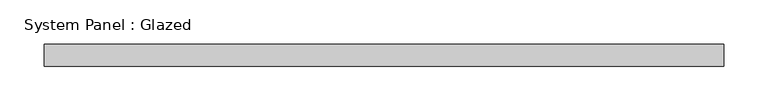
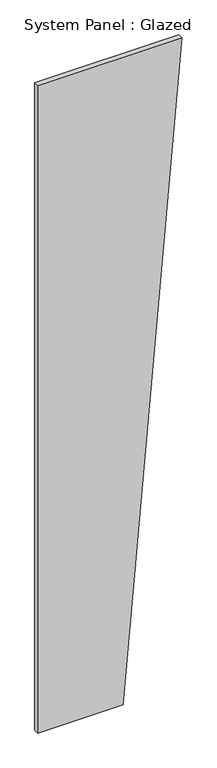
"""IFC4 building model written with IfcOpenShell, lengths in millimetres: plate geometry, System Panel : Glazed."""

import ifcopenshell
import ifcopenshell.guid

model = None  # the IFC model being written
_history = None  # IfcOwnerHistory: only IFC2X3 demands one
_inside = {}  # id of a spatial element -> (the spatial element, [elements in it])
_under = {}  # id of a project, library or spatial element -> (it, [spatial elements below it])
_declared = {}  # id of a project -> (the project, [libraries it declares])
_typed = {}  # id of a type object -> (the type object, [elements of that type])
_made_of = {}  # id of a material, layer set ... -> (it, [elements and type objects made of it])


def new_model(schema):
    """Start an empty IFC model of exactly this schema.

    Asked for "IFC4X3", IfcOpenShell would pick the latest addendum, in which some entities
    have other attributes; the version numbers below select the first issue.
    IFC2X3 requires an IfcOwnerHistory on every rooted entity: one is made here for all.
    """
    global model, _history
    if schema == "IFC4X3":
        model = ifcopenshell.file(schema_version=(4, 3, 0, 0))
    else:
        model = ifcopenshell.file(schema=schema)
    _inside.clear()
    _under.clear()
    _declared.clear()
    _typed.clear()
    _made_of.clear()
    _history = None
    if model.schema == "IFC2X3":
        org = make("IfcOrganization", Name="unknown")
        user = make(
            "IfcPersonAndOrganization",
            ThePerson=make("IfcPerson", FamilyName="unknown"),
            TheOrganization=org,
        )
        app = make(
            "IfcApplication",
            ApplicationDeveloper=org,
            Version="unknown",
            ApplicationFullName="unknown",
            ApplicationIdentifier="unknown",
        )
        _history = make(
            "IfcOwnerHistory",
            OwningUser=user,
            OwningApplication=app,
            ChangeAction="ADDED",
            CreationDate=0,
        )
    return model


def make(cls, **values):
    """One entity of the class cls with the attributes given. An attribute that is None is left unset."""
    return model.create_entity(
        cls, **{name: value for name, value in values.items() if value is not None}
    )


def rooted(cls, **values):
    """An entity with a GlobalId (a new one), such as an element, a storey or a relation."""
    return make(cls, GlobalId=ifcopenshell.guid.new(), OwnerHistory=_history, **values)


def si_unit(unit_type, name, prefix=None):
    """IfcSIUnit, for example si_unit("LENGTHUNIT", "METRE", prefix="MILLI")."""
    return make("IfcSIUnit", UnitType=unit_type, Prefix=prefix, Name=name)


def assignment(units):
    """IfcUnitAssignment: the units of a project."""
    return None if units is None else make("IfcUnitAssignment", Units=units)


def point(xyz):
    """IfcCartesianPoint."""
    return None if xyz is None else make("IfcCartesianPoint", Coordinates=xyz)


def direction(xyz):
    """IfcDirection."""
    return None if xyz is None else make("IfcDirection", DirectionRatios=xyz)


def frame(location, z_axis=None, x_axis=None):
    """IfcAxis2Placement3D, a coordinate frame: its origin and axes. An axis left out is left unset."""
    return make(
        "IfcAxis2Placement3D",
        Location=point(location),
        Axis=direction(z_axis),
        RefDirection=direction(x_axis),
    )


def origin():
    """The frame at (0, 0, 0) with its axes left unset."""
    return frame((0.0, 0.0, 0.0))


def place(relative_to, where):
    """IfcLocalPlacement: puts the frame where relative to a parent placement (None: the world)."""
    return make(
        "IfcLocalPlacement", PlacementRelTo=relative_to, RelativePlacement=where
    )


def context(
    kind, dimensions, precision=None, world=None, true_north=None, identifier=None
):
    """IfcGeometricRepresentationContext, for example the 3D "Model" context."""
    return make(
        "IfcGeometricRepresentationContext",
        ContextIdentifier=identifier,
        ContextType=kind,
        CoordinateSpaceDimension=dimensions,
        Precision=precision,
        WorldCoordinateSystem=world,
        TrueNorth=true_north,
    )


def project(units=None, contexts=None):
    """IfcProject with its units and contexts."""
    return rooted(
        "IfcProject",
        Name="project",
        RepresentationContexts=contexts,
        UnitsInContext=assignment(units),
    )


def spatial(cls, under=None, at=None, **own):
    """A site, building, storey or space (cls), placed at a placement, below another one or the project."""
    s = rooted(cls, ObjectPlacement=at, **own)
    if under is not None:
        _under.setdefault(under.id(), (under, []))[1].append(s)
    return s


def polyline(points):
    """IfcPolyline through the points."""
    return make("IfcPolyline", Points=[point(p) for p in points])


def outline(outer, holes=None, kind="AREA"):
    """IfcArbitraryClosedProfileDef: a profile drawn as a closed curve; with holes, ...WithVoids."""
    if holes is None:
        return make("IfcArbitraryClosedProfileDef", ProfileType=kind, OuterCurve=outer)
    return make(
        "IfcArbitraryProfileDefWithVoids",
        ProfileType=kind,
        OuterCurve=outer,
        InnerCurves=holes,
    )


def extrude(swept, where, along, depth):
    """IfcExtrudedAreaSolid: the profile swept, set in the frame where, extruded along a direction by depth."""
    return make(
        "IfcExtrudedAreaSolid",
        SweptArea=swept,
        Position=where,
        ExtrudedDirection=direction(along),
        Depth=depth,
    )


def shape(context_of_items, identifier, shape_type, items):
    """IfcShapeRepresentation: the items that make up one representation, for example the "Body"."""
    return make(
        "IfcShapeRepresentation",
        ContextOfItems=context_of_items,
        RepresentationIdentifier=identifier,
        RepresentationType=shape_type,
        Items=items,
    )


def source(mapping_origin, context_of_items, identifier, shape_type, items):
    """IfcRepresentationMap: a shape defined once, which mapped items show again and again."""
    return make(
        "IfcRepresentationMap",
        MappingOrigin=mapping_origin,
        MappedRepresentation=shape(context_of_items, identifier, shape_type, items),
    )


def transform(
    local_origin,
    x_axis=None,
    y_axis=None,
    z_axis=None,
    scale=None,
    scale2=None,
    scale3=None,
    uniform=True,
):
    """IfcCartesianTransformationOperator3D, or its non-uniform kind. x_axis, y_axis, z_axis: its Axis1, 2, 3."""
    if uniform:
        return make(
            "IfcCartesianTransformationOperator3D",
            Axis1=direction(x_axis),
            Axis2=direction(y_axis),
            LocalOrigin=point(local_origin),
            Scale=scale,
            Axis3=direction(z_axis),
        )
    return make(
        "IfcCartesianTransformationOperator3DnonUniform",
        Axis1=direction(x_axis),
        Axis2=direction(y_axis),
        LocalOrigin=point(local_origin),
        Scale=scale,
        Axis3=direction(z_axis),
        Scale2=scale2,
        Scale3=scale3,
    )


def mapped(mapping_source, mapping_target):
    """IfcMappedItem: shows the shape of a source again, moved by a transform."""
    return make(
        "IfcMappedItem", MappingSource=mapping_source, MappingTarget=mapping_target
    )


def made_of(thing, what):
    """Note that an element or type object is made of a material, layer set ...; save() writes the relation."""
    if what is not None:
        _made_of.setdefault(what.id(), (what, []))[1].append(thing)
    return thing


def element(
    cls,
    number,
    at=None,
    inside=None,
    cuts=None,
    type_object=None,
    material=None,
    context=None,
    identifier="Body",
    shape_type=None,
    held_by="IfcProductDefinitionShape",
    body=None,
    shapes=None,
    **own,
):
    """One element of the class cls, such as IfcWall. Its Tag is "e" and its number.

    at: its placement. inside: the storey or other place that contains it. cuts: it is an
    opening in that element (IfcRelVoidsElement). A single representation is given by context,
    identifier, shape_type and body (its items); several are given by shapes. held_by: the class
    of the entity that holds the representations. save() writes the other relations.
    """
    e = rooted(cls, Tag="e%d" % number, ObjectPlacement=at, **own)
    if body is not None:
        shapes = [shape(context, identifier, shape_type, body)]
    if shapes is not None:
        e.Representation = make(held_by, Representations=shapes)
    if inside is not None:
        _inside.setdefault(inside.id(), (inside, []))[1].append(e)
    if cuts is not None:
        rooted(
            "IfcRelVoidsElement", RelatingBuildingElement=cuts, RelatedOpeningElement=e
        )
    if type_object is not None:
        _typed.setdefault(type_object.id(), (type_object, []))[1].append(e)
    return made_of(e, material)


def aggregate(whole, parts):
    """IfcRelAggregates: a whole, such as a stair, and the parts it consists of."""
    return rooted("IfcRelAggregates", RelatingObject=whole, RelatedObjects=parts)


def save(model, path):
    """Write the relations noted so far, then the file.

    IfcRelAggregates (storeys below a building ...), IfcRelContainedInSpatialStructure (elements
    in a storey), IfcRelDefinesByType, IfcRelAssociatesMaterial and IfcRelDeclares: one each for
    every whole, place, type object, material and project.
    """
    for whole, parts in _under.values():
        aggregate(whole, parts)
    for where, things in _inside.values():
        rooted(
            "IfcRelContainedInSpatialStructure",
            RelatedElements=things,
            RelatingStructure=where,
        )
    for kind, things in _typed.values():
        rooted("IfcRelDefinesByType", RelatedObjects=things, RelatingType=kind)
    for what, things in _made_of.values():
        rooted("IfcRelAssociatesMaterial", RelatedObjects=things, RelatingMaterial=what)
    for by, libraries in _declared.values():
        rooted("IfcRelDeclares", RelatingContext=by, RelatedDefinitions=libraries)
    model.write(path)


def system_panel_glazed_ca25d662(model_context):
    return source(origin(), model_context, "Body", "SweptSolid", [
        extrude(outline(polyline([(0.0, -386.1685195), (0.0, 71.0314805), (3657.6, 386.1685195), (3657.6, -386.1685195), (0.0, -386.1685195)])), frame((0.0, -44.45, 0.0), z_axis=(0.0, 1.0, 0.0), x_axis=(0.0, 0.0, 1.0)), (0.0, 0.0, 1.0), 25.4),
    ])


if __name__ == "__main__":
    model = new_model("IFC4")
    model_context = context("Model", 3, world=origin())
    ifc_project = project(units=[si_unit("LENGTHUNIT", "METRE", prefix="MILLI")], contexts=[model_context])
    site = spatial("IfcSite", under=ifc_project)
    building = spatial("IfcBuilding", under=site)
    placement = place(None, origin())
    system_panel_glazed_shape = system_panel_glazed_ca25d662(model_context)
    element("IfcPlate", 1, ObjectType="System Panel : Glazed", at=placement, inside=building, context=model_context, shape_type="MappedRepresentation", body=[
        mapped(system_panel_glazed_shape, transform((0.0, 0.0, 0.0), x_axis=(1.0, 0.0, 0.0), y_axis=(0.0, 1.0, 0.0), z_axis=(0.0, 0.0, 1.0))),
    ])
    save(model, "model.ifc")

# Revit data of these elements
# Type "System Panel : Glazed"
#   Construction Type Id = "GSP4R"
#   Analytic Construction = "1/8 in Pilkington single glazing"
#   Visual Light Transmittance = 0.9
#   Solar Heat Gain Coefficient = 0.86
#   Heat Transfer Coefficient (U) = 1.18115 BTU/(h·ft²·°F)
#   Define Thermal Properties by = 1
# Element 1 (IfcPlate, "System Panel : Glazed")
#   Materials on its faces: "Glass"
# Materials
#   "Glass": class "Glass", colour RGB 0 128 192, transparency 0.75, Description = "Soda Lime Glass", Cost = 0
